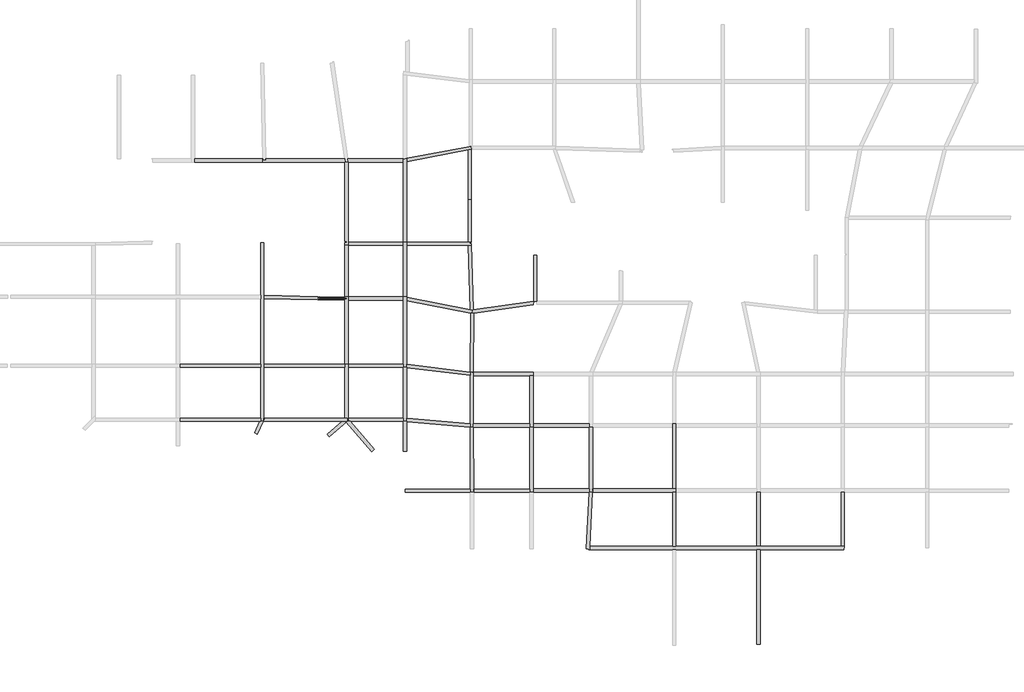
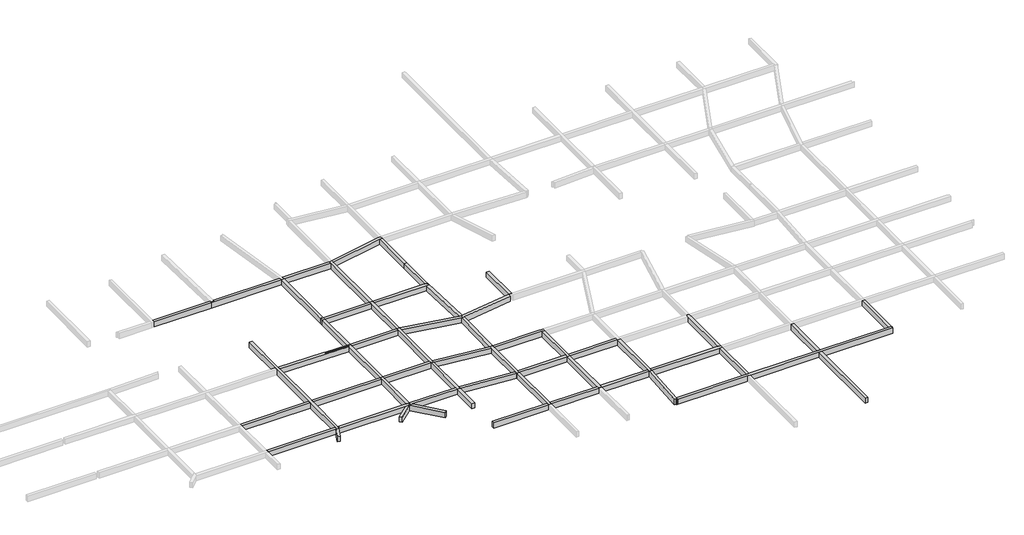
# One storey, part 3 of 15: 55 beams.
"""IFC4 building model written with IfcOpenShell, lengths in millimetres."""

from ifc_helpers import new_model, si_unit, frame, origin, place, context, project, spatial, polyline, outline, extrude, faceted_brep, element, save

model = new_model("IFC4")

# Units and contexts
model_context = context("Model", 3, world=origin())
ifc_project = project(units=[si_unit("LENGTHUNIT", "METRE", prefix="MILLI")], contexts=[model_context])

# Site, building, storey
site = spatial("IfcSite", under=ifc_project)
building = spatial("IfcBuilding", under=site)
storey = spatial("IfcBuildingStorey", under=building, Name="层高", Elevation=3300.0)

# Beams
placement = place(None, origin())
element("IfcBeam", 1, ObjectType="混凝土 - 矩形梁 : KL_beam", at=placement, inside=storey, context=model_context, shape_type="Brep", body=[
    faceted_brep([(134350.2032763, 38806.8951488, 3300.0), (134596.9927787, 38806.8951488, 3300.0), (134650.2032763, 38806.8951488, 3300.0), (134650.2032763, 38924.5535194, 3300.0), (134650.2032763, 39106.8951488, 3300.0), (134650.2032763, 43792.5925365, 3300.0), (134650.2032763, 44092.5925365, 3300.0), (134650.2032763, 50164.3231436, 3300.0), (134650.2032763, 50464.3928831, 3300.0), (134650.2032763, 55332.5925367, 3300.0), (134350.2032763, 55332.5925367, 3300.0), (134350.2032763, 50467.5925366, 3300.0), (134350.2032763, 50167.5925366, 3300.0), (134350.2032763, 44092.5925365, 3300.0), (134350.2032763, 43792.5925365, 3300.0), (134350.2032763, 39106.8951488, 3300.0), (134650.2032763, 38806.8951488, 2700.0), (134650.2032763, 38924.5535194, 2700.0), (134650.2032763, 39106.8951488, 2700.0), (134650.2032763, 43792.5925365, 2700.0), (134650.2032763, 44092.5925365, 2700.0), (134650.2032763, 50164.3231436, 2700.0), (134650.2032763, 50464.3928831, 2700.0), (134650.2032763, 55332.5925367, 2700.0), (134596.9927787, 38806.8951488, 2700.0), (134350.2032763, 38806.8951488, 2700.0), (134350.2032763, 39106.8951488, 2700.0), (134350.2032763, 43792.5925365, 2700.0), (134350.2032763, 44092.5925365, 2700.0), (134350.2032763, 50167.5925366, 2700.0), (134350.2032763, 50467.5925366, 2700.0), (134350.2032763, 55332.5925367, 2700.0)], [[[0, 1, 2, 3, 4, 5, 6, 7, 8, 9, 10, 11, 12, 13, 14, 15]], [[2, 16, 17, 18, 19, 20, 21, 22, 23, 9, 8, 7, 6, 5, 4, 3]], [[16, 24, 25, 26, 27, 28, 29, 30, 31, 23, 22, 21, 20, 19, 18, 17]], [[25, 0, 15, 14, 13, 12, 11, 10, 31, 30, 29, 28, 27, 26]], [[2, 1, 0, 25, 24, 16]], [[10, 9, 23, 31]]]),
])
element("IfcBeam", 2, ObjectType="混凝土 - 矩形梁 : KL_beam", at=placement, inside=storey, context=model_context, shape_type="SweptSolid", body=[
    extrude(outline(polyline([(134350.2032763, 44092.5925365), (134350.2032763, 43792.5925365), (126850.2032763, 43792.5925365), (126850.2032763, 44092.5925365), (134350.2032763, 44092.5925365)])), frame((0.0, 0.0, 2700.0), z_axis=(0.0, 0.0, 1.0), x_axis=(1.0, 0.0, 0.0)), (0.0, 0.0, 1.0), 600.0),
])
element("IfcBeam", 3, ObjectType="混凝土 - 矩形梁 : KL_beam", at=placement, inside=storey, context=model_context, shape_type="Brep", body=[
    faceted_brep([(134350.2032763, 38806.8951488, 3300.0), (134350.2032763, 39106.8951488, 3300.0), (126850.2032763, 39106.8951488, 3300.0), (126850.2032763, 38806.8951488, 3300.0), (134267.7400501, 38806.8951488, 3300.0), (134350.2032763, 38806.8951488, 2700.0), (126850.2032763, 38806.8951488, 2700.0), (134267.7400501, 38806.8951488, 2700.0), (134350.2032763, 39106.8951488, 2700.0), (126850.2032763, 39106.8951488, 2700.0)], [[[0, 1, 2, 3, 4]], [[5, 0, 4, 3, 6, 7]], [[8, 5, 7, 6, 9]], [[1, 8, 9, 2]], [[1, 0, 5, 8]], [[3, 2, 9, 6]]]),
])
element("IfcBeam", 4, ObjectType="混凝土 - 矩形梁 : KL_beam", at=placement, inside=storey, context=model_context, shape_type="Brep", body=[
    faceted_brep([(134060.3828953, 37620.3502485, 3300.0), (133787.0366413, 37743.969929, 3300.0), (133787.0366413, 37743.969929, 2700.0), (134060.3828953, 37620.3502485, 2700.0), (134596.9927787, 38806.8951488, 3300.0), (134350.2032763, 38806.8951488, 3300.0), (134267.7400501, 38806.8951488, 3300.0), (134267.7400501, 38806.8951488, 2700.0), (134350.2032763, 38806.8951488, 2700.0), (134596.9927787, 38806.8951488, 2700.0)], [[[0, 1, 2, 3]], [[1, 0, 4, 5, 6]], [[2, 1, 6, 7]], [[3, 2, 7, 8, 9]], [[0, 3, 9, 4]], [[4, 9, 8, 7, 6, 5]]]),
    faceted_brep([(134650.2032763, 39106.8951488, 2700.0), (134650.2032763, 39106.8951488, 3300.0), (134732.6665025, 39106.8951488, 3300.0), (134732.6665025, 39106.8951488, 2700.0), (134650.2032763, 38924.5535194, 3300.0), (134650.2032763, 38924.5535194, 2700.0)], [[[0, 1, 2, 3]], [[4, 1, 0, 5]], [[4, 2, 1]], [[3, 5, 0]], [[2, 4, 5, 3]]]),
])
element("IfcBeam", 5, ObjectType="混凝土 - 矩形梁 : KL_beam", at=placement, inside=storey, context=model_context, shape_type="Brep", body=[
    faceted_brep([(142355.6857455, 38806.8951488, 3300.0), (142355.6857455, 39106.8951488, 3300.0), (142150.2032763, 39106.8951488, 3300.0), (134732.6665025, 39106.8951488, 3300.0), (134650.2032763, 38924.5535194, 3300.0), (134650.2032763, 38806.8951488, 3300.0), (141894.6697749, 38806.8951488, 3300.0), (142355.6857455, 38806.8951488, 2700.0), (134650.2032763, 38806.8951488, 2700.0), (141894.6697749, 38806.8951488, 2700.0), (142355.6857455, 39106.8951488, 2700.0), (134650.2032763, 38924.5535194, 2700.0), (134732.6665025, 39106.8951488, 2700.0), (142150.2032763, 39106.8951488, 2700.0)], [[[0, 1, 2, 3, 4, 5, 6]], [[7, 0, 6, 5, 8, 9]], [[10, 7, 9, 8, 11, 12, 13]], [[12, 3, 2, 1, 10, 13]], [[3, 12, 11, 4]], [[1, 0, 7, 10]], [[5, 4, 11, 8]]]),
])
element("IfcBeam", 6, ObjectType="混凝土 - 矩形梁 : KL_beam", at=placement, inside=storey, context=model_context, shape_type="SweptSolid", body=[
    extrude(outline(polyline([(140719.4659799, 37404.6255236), (140524.2449773, 37632.4165685), (141894.6697749, 38806.8951488), (142355.6857455, 38806.8951488), (140719.4659799, 37404.6255236)])), frame((0.0, 0.0, 2700.0), z_axis=(0.0, 0.0, 1.0), x_axis=(1.0, 0.0, 0.0)), (0.0, 0.0, 1.0), 600.0),
])
element("IfcBeam", 7, ObjectType="混凝土 - 矩形梁 : KL_beam", at=placement, inside=storey, context=model_context, shape_type="Brep", body=[
    faceted_brep([(142450.2032763, 44092.5925365, 3300.0), (142150.2032763, 44092.5925365, 3300.0), (142150.2032763, 43792.5925365, 3300.0), (142150.2032763, 39106.8951488, 3300.0), (142244.7208071, 39106.8951488, 3300.0), (142355.6857455, 39106.8951488, 3300.0), (142355.6857455, 38806.8951488, 3300.0), (142450.2032763, 38806.8951488, 3300.0), (142450.2032763, 39106.8951488, 3300.0), (142450.2032763, 43792.5925365, 3300.0), (142150.2032763, 39106.8951488, 2700.0), (142150.2032763, 44092.5925365, 2700.0), (142150.2032763, 43792.5925365, 2700.0), (142450.2032763, 44092.5925365, 2700.0), (142450.2032763, 43792.5925365, 2700.0), (142450.2032763, 39106.8951488, 2700.0), (142450.2032763, 38806.8951488, 2700.0), (142355.6857455, 38806.8951488, 2700.0), (142355.6857455, 39106.8951488, 2700.0), (142244.7208071, 39106.8951488, 2700.0)], [[[0, 1, 2, 3, 4, 5, 6, 7, 8, 9]], [[10, 3, 2, 1, 11, 12]], [[11, 13, 14, 15, 16, 17, 18, 19, 10, 12]], [[7, 16, 15, 14, 13, 0, 9, 8]], [[16, 7, 6, 17]], [[3, 10, 19, 18, 5, 4]], [[1, 0, 13, 11]], [[5, 18, 17, 6]]]),
])
element("IfcBeam", 8, ObjectType="混凝土 - 矩形梁 : KL_beam", at=placement, inside=storey, context=model_context, shape_type="SweptSolid", body=[
    extrude(outline(polyline([(142150.2032763, 44092.5925365), (142150.2032763, 43792.5925365), (134650.2032763, 43792.5925365), (134650.2032763, 44092.5925365), (142150.2032763, 44092.5925365)])), frame((0.0, 0.0, 2700.0), z_axis=(0.0, 0.0, 1.0), x_axis=(1.0, 0.0, 0.0)), (0.0, 0.0, 1.0), 600.0),
])
element("IfcBeam", 9, ObjectType="混凝土 - 矩形梁 : KL_beam", at=placement, inside=storey, context=model_context, shape_type="Brep", body=[
    faceted_brep([(142150.2032763, 44092.5925365, 3300.0), (142450.2032763, 44092.5925365, 3300.0), (142450.2032763, 50017.6336553, 3300.0), (142450.2032763, 50317.6336553, 3300.0), (142150.2032763, 50317.6336553, 3300.0), (142150.2032763, 50302.6667178, 3300.0), (142150.2032763, 50227.6336553, 3300.0), (142300.2032763, 50227.6336553, 3300.0), (142300.2032763, 50107.6336553, 3300.0), (142150.2032763, 50107.6336553, 3300.0), (142150.2032763, 50002.5969783, 3300.0), (142450.2032763, 44092.5925365, 2700.0), (142450.2032763, 50017.6336553, 2700.0), (142450.2032763, 50317.6336553, 2700.0), (142150.2032763, 44092.5925365, 2700.0), (142150.2032763, 50002.5969783, 2700.0), (142150.2032763, 50107.6336553, 2700.0), (142300.2032763, 50107.6336553, 2700.0), (142300.2032763, 50227.6336553, 2700.0), (142150.2032763, 50227.6336553, 2700.0), (142150.2032763, 50302.6667178, 2700.0), (142150.2032763, 50317.6336553, 2700.0)], [[[0, 1, 2, 3, 4, 5, 6, 7, 8, 9, 10]], [[1, 11, 12, 13, 3, 2]], [[11, 14, 15, 16, 17, 18, 19, 20, 21, 13, 12]], [[14, 0, 10, 9, 16, 15]], [[1, 0, 14, 11]], [[4, 3, 13, 21]], [[8, 17, 16, 9]], [[18, 7, 6, 19]], [[17, 8, 7, 18]], [[4, 21, 20, 19, 6, 5]]]),
])
element("IfcBeam", 10, ObjectType="混凝土 - 矩形梁 : KL_beam", at=placement, inside=storey, context=model_context, shape_type="SweptSolid", body=[
    extrude(outline(polyline([(139760.2139729, 50227.6336553), (139760.2139729, 50354.2032252), (142150.2032763, 50302.6667178), (142150.2032763, 50227.6336553), (139760.2139729, 50227.6336553)])), frame((0.0, 0.0, 2700.0), z_axis=(0.0, 0.0, 1.0), x_axis=(1.0, 0.0, 0.0)), (0.0, 0.0, 1.0), 600.0),
    extrude(outline(polyline([(134650.2032763, 50164.3231436), (134650.2032763, 50464.3928831), (139640.2139729, 50356.7908438), (139640.2139729, 50107.6336553), (142150.2032763, 50107.6336553), (142150.2032763, 50002.5969783), (134650.2032763, 50164.3231436)])), frame((0.0, 0.0, 2700.0), z_axis=(0.0, 0.0, 1.0), x_axis=(1.0, 0.0, 0.0)), (0.0, 0.0, 1.0), 600.0),
])
element("IfcBeam", 11, ObjectType="混凝土 - 矩形梁 : KL_beam", at=placement, inside=storey, context=model_context, shape_type="Brep", body=[
    faceted_brep([(147550.2032763, 43792.5925365, 3300.0), (147850.2032763, 43792.5925365, 3300.0), (147850.2032763, 44075.472827, 3300.0), (147850.2032763, 49985.080878, 3300.0), (147850.2032763, 50290.8856831, 3300.0), (147850.2032763, 50317.6336548, 3300.0), (147550.2032763, 50317.6336549, 3300.0), (147550.2032763, 50017.6336549, 3300.0), (147550.2032763, 44092.5925365, 3300.0), (147550.2032763, 43792.5925365, 2700.0), (147550.2032763, 50317.6336549, 2700.0), (147550.2032763, 50017.6336549, 2700.0), (147550.2032763, 44092.5925365, 2700.0), (147850.2032763, 43792.5925365, 2700.0), (147850.2032763, 50317.6336548, 2700.0), (147850.2032763, 50290.8856831, 2700.0), (147850.2032763, 49985.080878, 2700.0), (147850.2032763, 44075.472827, 2700.0)], [[[0, 1, 2, 3, 4, 5, 6, 7, 8]], [[9, 0, 8, 7, 6, 10, 11, 12]], [[13, 9, 12, 11, 10, 14, 15, 16, 17]], [[1, 13, 17, 16, 15, 14, 5, 4, 3, 2]], [[1, 0, 9, 13]], [[6, 5, 14, 10]]]),
])
element("IfcBeam", 12, ObjectType="混凝土 - 矩形梁 : KL_beam", at=placement, inside=storey, context=model_context, shape_type="SweptSolid", body=[
    extrude(outline(polyline([(142450.2032763, 43792.5925365), (142450.2032763, 44092.5925365), (147550.2032763, 44092.5925365), (147550.2032763, 43792.5925365), (142450.2032763, 43792.5925365)])), frame((0.0, 0.0, 2700.0), z_axis=(0.0, 0.0, 1.0), x_axis=(1.0, 0.0, 0.0)), (0.0, 0.0, 1.0), 600.0),
])
element("IfcBeam", 13, ObjectType="混凝土 - 矩形梁 : KL_beam", at=placement, inside=storey, context=model_context, shape_type="Brep", body=[
    faceted_brep([(147550.2032763, 38806.8951488, 3300.0), (147850.2032763, 38806.8951488, 3300.0), (147850.2032763, 39094.3896048, 3300.0), (147850.2032763, 43773.2671993, 3300.0), (147850.2032763, 43792.5925365, 3300.0), (147550.2032763, 43792.5925365, 3300.0), (147550.2032763, 39106.8951488, 3300.0), (147550.2032763, 38806.8951488, 2700.0), (147550.2032763, 43792.5925365, 2700.0), (147550.2032763, 39106.8951488, 2700.0), (147850.2032763, 38806.8951488, 2700.0), (147850.2032763, 43792.5925365, 2700.0), (147850.2032763, 43773.2671993, 2700.0), (147850.2032763, 39094.3896048, 2700.0)], [[[0, 1, 2, 3, 4, 5, 6]], [[7, 0, 6, 5, 8, 9]], [[10, 7, 9, 8, 11, 12, 13]], [[1, 10, 13, 12, 11, 4, 3, 2]], [[5, 4, 11, 8]], [[1, 0, 7, 10]]]),
])
element("IfcBeam", 14, ObjectType="混凝土 - 矩形梁 : KL_beam", at=placement, inside=storey, context=model_context, shape_type="Brep", body=[
    faceted_brep([(147550.2032763, 38806.8951488, 3300.0), (147550.2032763, 39106.8951488, 3300.0), (142450.2032763, 39106.8951488, 3300.0), (142450.2032763, 38806.8951488, 3300.0), (142626.6879476, 38806.8951488, 3300.0), (147550.2032763, 38806.8951488, 2700.0), (142450.2032763, 38806.8951488, 2700.0), (142626.6879476, 38806.8951488, 2700.0), (147550.2032763, 39106.8951488, 2700.0), (142450.2032763, 39106.8951488, 2700.0)], [[[0, 1, 2, 3, 4]], [[5, 0, 4, 3, 6, 7]], [[8, 5, 7, 6, 9]], [[1, 8, 9, 2]], [[1, 0, 5, 8]], [[3, 2, 9, 6]]]),
])
element("IfcBeam", 15, ObjectType="混凝土 - 矩形梁 : KL_beam", at=placement, inside=storey, context=model_context, shape_type="Brep", body=[
    faceted_brep([(147850.2032763, 36044.6279155, 3300.0), (147550.2032763, 36044.6279155, 3300.0), (147550.2032763, 36044.6279155, 2700.0), (147850.2032763, 36044.6279155, 2700.0), (147850.2032763, 38793.252187, 3300.0), (147850.2032763, 38806.8951488, 3300.0), (147550.2032763, 38806.8951488, 3300.0), (147550.2032763, 38806.8951488, 2700.0), (147850.2032763, 38806.8951488, 2700.0), (147850.2032763, 38793.252187, 2700.0)], [[[0, 1, 2, 3]], [[1, 0, 4, 5, 6]], [[2, 1, 6, 7]], [[3, 2, 7, 8, 9]], [[0, 3, 9, 8, 5, 4]], [[6, 5, 8, 7]]]),
])
element("IfcBeam", 16, ObjectType="混凝土 - 矩形梁 : KL_beam", at=placement, inside=storey, context=model_context, shape_type="Brep", body=[
    faceted_brep([(144852.3235863, 36214.6134538, 3300.0), (144624.7063393, 36019.1898399, 3300.0), (144624.7063393, 36019.1898399, 2700.0), (144852.3235863, 36214.6134538, 2700.0), (142626.6879476, 38806.8951488, 3300.0), (142450.2032763, 38806.8951488, 3300.0), (142355.6857455, 38806.8951488, 3300.0), (142284.0195543, 38745.4759403, 3300.0), (142284.0195543, 38745.4759403, 2700.0), (142355.6857455, 38806.8951488, 2700.0), (142450.2032763, 38806.8951488, 2700.0), (142626.6879476, 38806.8951488, 2700.0)], [[[0, 1, 2, 3]], [[1, 0, 4, 5, 6, 7]], [[2, 1, 7, 8]], [[3, 2, 8, 9, 10, 11]], [[0, 3, 11, 4]], [[7, 6, 9, 8]], [[4, 11, 10, 9, 6, 5]]]),
])
element("IfcBeam", 17, ObjectType="混凝土 - 矩形梁 : KL_beam", at=placement, inside=storey, context=model_context, shape_type="Brep", body=[
    faceted_brep([(154026.6104044, 43325.1413406, 3300.0), (153885.7263771, 43342.2564237, 3300.0), (153728.3021275, 43361.3808708, 3300.0), (153726.6104044, 43361.5863872, 3300.0), (153726.6104044, 43059.3807595, 3300.0), (153726.6104044, 38582.19205, 3300.0), (153726.6104044, 38281.0546322, 3300.0), (153726.6104044, 38266.5295438, 3300.0), (153727.1862138, 38266.5295438, 3300.0), (154026.6104044, 38266.5295438, 3300.0), (154026.6104044, 38566.5295438, 3300.0), (154026.6104044, 43042.1845858, 3300.0), (154026.6104044, 43325.1413406, 2700.0), (154026.6104044, 38266.5295438, 2700.0), (154026.6104044, 38566.5295438, 2700.0), (154026.6104044, 43042.1845858, 2700.0), (153726.6104044, 43361.5863872, 2700.0), (153728.3021275, 43361.3808708, 2700.0), (153885.7263771, 43342.2564237, 2700.0), (153727.1862138, 38266.5295438, 2700.0), (153726.6104044, 38266.5295438, 2700.0), (153726.6104044, 38281.0546322, 2700.0), (153726.6104044, 38582.19205, 2700.0), (153726.6104044, 43059.3807595, 2700.0)], [[[0, 1, 2, 3, 4, 5, 6, 7, 8, 9, 10, 11]], [[12, 0, 11, 10, 9, 13, 14, 15]], [[16, 17, 18, 12, 15, 14, 13, 19, 20, 21, 22, 23]], [[3, 16, 23, 22, 21, 20, 7, 6, 5, 4]], [[3, 2, 1, 0, 12, 18, 17, 16]], [[9, 8, 7, 20, 19, 13]]]),
])
element("IfcBeam", 18, ObjectType="混凝土 - 矩形梁 : KL_beam", at=placement, inside=storey, context=model_context, shape_type="Brep", body=[
    faceted_brep([(147850.2032763, 44075.472827, 3300.0), (147850.2032763, 43792.5925365, 3300.0), (147850.2032763, 43773.2671993, 3300.0), (153726.6104044, 43059.3807595, 3300.0), (153726.6104044, 43361.5863872, 3300.0), (147850.2032763, 43773.2671993, 2700.0), (153726.6104044, 43059.3807595, 2700.0), (147850.2032763, 43792.5925365, 2700.0), (147850.2032763, 44075.472827, 2700.0), (153726.6104044, 43361.5863872, 2700.0)], [[[0, 1, 2, 3, 4]], [[2, 5, 6, 3]], [[5, 7, 8, 9, 6]], [[8, 0, 4, 9]], [[0, 8, 7, 5, 2, 1]], [[4, 3, 6, 9]]]),
])
element("IfcBeam", 19, ObjectType="混凝土 - 矩形梁 : KL_beam", at=placement, inside=storey, context=model_context, shape_type="Brep", body=[
    faceted_brep([(159549.7804968, 43039.3698021, 3300.0), (159549.7804968, 43042.2492414, 3300.0), (159549.7804968, 43185.5183781, 3300.0), (159549.7804968, 43339.3698411, 3300.0), (159257.4396146, 43339.5188273, 3300.0), (154028.1243818, 43342.1838531, 3300.0), (153885.7263771, 43342.2564237, 3300.0), (154026.6104044, 43325.1413406, 3300.0), (154026.6104044, 43042.1845858, 3300.0), (159248.1480987, 43039.5235236, 3300.0), (159249.7804968, 43039.5226917, 3300.0), (159549.7804968, 43039.3698021, 2700.0), (154026.6104044, 43042.1845858, 2700.0), (159248.1480987, 43039.5235236, 2700.0), (159249.7804968, 43039.5226917, 2700.0), (159549.7804968, 43339.3698411, 2700.0), (159549.7804968, 43185.5183781, 2700.0), (159549.7804968, 43042.2492414, 2700.0), (154026.6104044, 43325.1413406, 2700.0), (153885.7263771, 43342.2564237, 2700.0), (154028.1243818, 43342.1838531, 2700.0), (159257.4396146, 43339.5188273, 2700.0)], [[[0, 1, 2, 3, 4, 5, 6, 7, 8, 9, 10]], [[11, 0, 10, 9, 8, 12, 13, 14]], [[15, 16, 17, 11, 14, 13, 12, 18, 19, 20, 21]], [[3, 15, 21, 20, 19, 6, 5, 4]], [[3, 2, 1, 0, 11, 17, 16, 15]], [[18, 7, 6, 19]], [[7, 18, 12, 8]]]),
])
element("IfcBeam", 20, ObjectType="混凝土 - 矩形梁 : KL_beam", at=placement, inside=storey, context=model_context, shape_type="Brep", body=[
    faceted_brep([(159249.7804968, 38266.5295438, 3300.0), (159549.7804968, 38266.5295438, 3300.0), (159549.7804968, 38566.5295438, 3300.0), (159549.7804968, 43039.3698021, 3300.0), (159249.7804968, 43039.5226917, 3300.0), (159249.7804968, 38566.5295438, 3300.0), (159249.7804968, 38266.5295438, 2700.0), (159249.7804968, 43039.5226917, 2700.0), (159249.7804968, 38566.5295438, 2700.0), (159549.7804968, 38266.5295438, 2700.0), (159549.7804968, 43039.3698021, 2700.0), (159549.7804968, 38566.5295438, 2700.0)], [[[0, 1, 2, 3, 4, 5]], [[6, 0, 5, 4, 7, 8]], [[9, 6, 8, 7, 10, 11]], [[1, 9, 11, 10, 3, 2]], [[4, 3, 10, 7]], [[1, 0, 6, 9]]]),
])
element("IfcBeam", 21, ObjectType="混凝土 - 矩形梁 : KL_beam", at=placement, inside=storey, context=model_context, shape_type="Brep", body=[
    faceted_brep([(159249.7804968, 38266.5295438, 3300.0), (159249.7804968, 38566.5295438, 3300.0), (154026.6104044, 38566.5295438, 3300.0), (154026.6104044, 38266.5295438, 3300.0), (154027.1884327, 38266.5295438, 3300.0), (159249.7804968, 38266.5295438, 2700.0), (154026.6104044, 38266.5295438, 2700.0), (154027.1884327, 38266.5295438, 2700.0), (159249.7804968, 38566.5295438, 2700.0), (154026.6104044, 38566.5295438, 2700.0)], [[[0, 1, 2, 3, 4]], [[5, 0, 4, 3, 6, 7]], [[8, 5, 7, 6, 9]], [[1, 8, 9, 2]], [[1, 0, 5, 8]], [[3, 2, 9, 6]]]),
])
element("IfcBeam", 22, ObjectType="混凝土 - 矩形梁 : KL_beam", at=placement, inside=storey, context=model_context, shape_type="Brep", body=[
    faceted_brep([(153750.3563062, 32242.26105, 3300.0), (154050.3540873, 32243.4148791, 3300.0), (154049.7804968, 32392.5495084, 3300.0), (154049.2046874, 32542.26105, 3300.0), (154027.1884327, 38266.5295438, 3300.0), (154026.6104044, 38266.5295438, 3300.0), (153727.1862138, 38266.5295438, 3300.0), (153749.2024685, 32542.26105, 3300.0), (154050.3540873, 32243.4148791, 2700.0), (154049.7804968, 32392.5495084, 2700.0), (154049.2046874, 32542.26105, 2700.0), (154027.1884327, 38266.5295438, 2700.0), (153750.3563062, 32242.26105, 2700.0), (153749.2024685, 32542.26105, 2700.0), (153727.1862138, 38266.5295438, 2700.0), (154026.6104044, 38266.5295438, 2700.0)], [[[0, 1, 2, 3, 4, 5, 6, 7]], [[1, 8, 9, 10, 11, 4, 3, 2]], [[8, 12, 13, 14, 15, 11, 10, 9]], [[12, 0, 7, 6, 14, 13]], [[6, 5, 4, 11, 15, 14]], [[0, 12, 8, 1]]]),
])
element("IfcBeam", 23, ObjectType="混凝土 - 矩形梁 : KL_beam", at=placement, inside=storey, context=model_context, shape_type="Brep", body=[
    faceted_brep([(147748.4611459, 32242.26105, 3300.0), (147748.4611459, 32542.26105, 3300.0), (147748.4611459, 32542.26105, 2700.0), (147748.4611459, 32242.26105, 2700.0), (153749.7804968, 32242.26105, 3300.0), (153750.3563062, 32242.26105, 3300.0), (153749.2024685, 32542.26105, 3300.0), (153749.2024685, 32542.26105, 2700.0), (153750.3563062, 32242.26105, 2700.0), (153749.7804968, 32242.26105, 2700.0), (154049.7804968, 32242.26105, 2700.0), (154050.3585251, 32242.26105, 2700.0), (154050.3585251, 32242.26105, 3300.0), (154049.7804968, 32242.26105, 3300.0), (154050.3540873, 32243.4148791, 2700.0), (154050.3540873, 32243.4148791, 3300.0)], [[[0, 1, 2, 3]], [[1, 0, 4, 5, 6]], [[2, 1, 6, 7]], [[3, 2, 7, 8, 9]], [[0, 3, 9, 8, 10, 11, 12, 13, 5, 4]], [[5, 8, 7, 6]], [[12, 11, 14, 15]], [[8, 5, 15, 14]], [[5, 13, 12, 15]], [[14, 11, 10, 8]]]),
])
element("IfcBeam", 24, ObjectType="混凝土 - 矩形梁 : KL_beam", at=placement, inside=storey, context=model_context, shape_type="SweptSolid", body=[
    extrude(outline(polyline([(142450.2032763, 50017.6336553), (142450.2032763, 50317.6336553), (147550.2032763, 50317.6336549), (147550.2032763, 50017.6336549), (142450.2032763, 50017.6336553)])), frame((0.0, 0.0, 2700.0), z_axis=(0.0, 0.0, 1.0), x_axis=(1.0, 0.0, 0.0)), (0.0, 0.0, 1.0), 600.0),
])
element("IfcBeam", 25, ObjectType="混凝土 - 矩形梁 : KL_beam", at=placement, inside=storey, context=model_context, shape_type="Brep", body=[
    faceted_brep([(147850.2032738, 55392.5925366, 3300.0), (147550.2032738, 55392.5925366, 3300.0), (147550.2032738, 55382.5925365, 3300.0), (147550.203274, 55082.5925365, 3300.0), (147550.2032762, 50317.6336549, 3300.0), (147850.2032762, 50317.6336548, 3300.0), (147850.203274, 55092.5925366, 3300.0), (147550.2032738, 55392.5925366, 2700.0), (147550.2032738, 55382.5925365, 2700.0), (147550.203274, 55082.5925365, 2700.0), (147550.2032762, 50317.6336549, 2700.0), (147850.2032738, 55392.5925366, 2700.0), (147850.203274, 55092.5925366, 2700.0), (147850.2032762, 50317.6336548, 2700.0)], [[[0, 1, 2, 3, 4, 5, 6]], [[1, 7, 8, 9, 10, 4, 3, 2]], [[7, 11, 12, 13, 10, 9, 8]], [[11, 0, 6, 5, 13, 12]], [[1, 0, 11, 7]], [[5, 4, 10, 13]]]),
])
element("IfcBeam", 26, ObjectType="混凝土 - 矩形梁 : KL_beam", at=placement, inside=storey, context=model_context, shape_type="Brep", body=[
    faceted_brep([(153895.7696272, 48790.0588433, 3300.0), (153903.7913665, 49094.2779979, 3300.0), (153721.7041547, 49130.2710244, 3300.0), (147850.2032762, 50290.8856831, 3300.0), (147850.2032762, 50017.6336548, 3300.0), (147850.2032763, 49985.080878, 3300.0), (153783.0726395, 48812.3355624, 3300.0), (147850.2032763, 49985.080878, 2700.0), (153783.0726395, 48812.3355624, 2700.0), (153895.7696272, 48790.0588433, 2700.0), (153903.7913665, 49094.2779979, 2700.0), (147850.2032762, 50017.6336548, 2700.0), (147850.2032762, 50290.8856831, 2700.0), (153721.7041547, 49130.2710244, 2700.0)], [[[0, 1, 2, 3, 4, 5, 6]], [[5, 7, 8, 9, 0, 6]], [[10, 9, 8, 7, 11, 12, 13]], [[12, 3, 2, 1, 10, 13]], [[3, 12, 11, 7, 5, 4]], [[1, 0, 9, 10]]]),
])
element("IfcBeam", 27, ObjectType="混凝土 - 矩形梁 : KL_beam", at=placement, inside=storey, context=model_context, shape_type="Brep", body=[
    faceted_brep([(147850.2032738, 55392.5925366, 3300.0), (147850.203274, 55092.5925366, 3300.0), (153554.4497163, 55092.5925366, 3300.0), (153850.3009381, 55092.5925366, 3300.0), (153850.3009381, 55244.6960153, 3300.0), (153850.3009381, 55257.9423641, 3300.0), (153700.298991, 55257.9423641, 3300.0), (153700.298991, 55377.9423641, 3300.0), (153850.3009381, 55377.9423641, 3300.0), (153850.3009381, 55392.5925366, 3300.0), (153550.3009381, 55392.5925366, 3300.0), (153850.3009381, 55092.5925366, 2700.0), (147850.203274, 55092.5925366, 2700.0), (153554.4497163, 55092.5925366, 2700.0), (147850.2032738, 55392.5925366, 2700.0), (153550.3009381, 55392.5925366, 2700.0), (153850.3009381, 55392.5925366, 2700.0), (153850.3009381, 55377.9423641, 2700.0), (153700.298991, 55377.9423641, 2700.0), (153700.298991, 55257.9423641, 2700.0), (153850.3009381, 55257.9423641, 2700.0), (153850.3009381, 55244.6960153, 2700.0)], [[[0, 1, 2, 3, 4, 5, 6, 7, 8, 9, 10]], [[11, 3, 2, 1, 12, 13]], [[12, 14, 15, 16, 17, 18, 19, 20, 21, 11, 13]], [[9, 16, 15, 14, 0, 10]], [[16, 9, 8, 17]], [[1, 0, 14, 12]], [[7, 18, 17, 8]], [[19, 6, 5, 20]], [[18, 7, 6, 19]], [[3, 11, 21, 20, 5, 4]]]),
])
element("IfcBeam", 28, ObjectType="混凝土 - 矩形梁 : KL_beam", at=placement, inside=storey, context=model_context, shape_type="SweptSolid", body=[
    extrude(outline(polyline([(153550.3009381, 59292.1684205), (153850.3009381, 59292.1684205), (153850.3009381, 55392.5925366), (153550.3009381, 55392.5925366), (153550.3009381, 59292.1684205)])), frame((0.0, 0.0, 2700.0), z_axis=(0.0, 0.0, 1.0), x_axis=(1.0, 0.0, 0.0)), (0.0, 0.0, 1.0), 600.0),
])
element("IfcBeam", 29, ObjectType="混凝土 - 矩形梁 : KL_beam", at=placement, inside=storey, context=model_context, shape_type="Brep", body=[
    faceted_brep([(147850.2032739, 63124.0584778, 3300.0), (147550.2032739, 63066.5805581, 3300.0), (147550.2032739, 62792.591237, 3300.0), (147550.2032739, 55392.5925366, 3300.0), (147850.2032739, 55392.5925366, 3300.0), (147850.2032739, 62818.6019158, 3300.0), (147850.2032739, 63124.0584778, 2700.0), (147850.2032739, 55392.5925366, 2700.0), (147850.2032739, 62818.6019158, 2700.0), (147550.2032739, 63066.5805581, 2700.0), (147550.2032739, 55392.5925366, 2700.0), (147550.2032739, 62792.591237, 2700.0)], [[[0, 1, 2, 3, 4, 5]], [[6, 0, 5, 4, 7, 8]], [[9, 6, 8, 7, 10, 11]], [[1, 9, 11, 10, 3, 2]], [[4, 3, 10, 7]], [[1, 0, 6, 9]]]),
])
element("IfcBeam", 30, ObjectType="混凝土 - 矩形梁 : KL_beam", at=placement, inside=storey, context=model_context, shape_type="Brep", body=[
    faceted_brep([(153850.3013477, 63968.1790994, 3300.0), (153793.8501921, 64262.8200114, 3300.0), (153625.2394262, 64230.5153579, 3300.0), (147850.2032739, 63124.0584778, 3300.0), (147850.2032739, 62818.6019158, 3300.0), (153550.3013477, 63910.7011797, 3300.0), (153793.8501921, 64262.8200114, 2700.0), (153625.2394262, 64230.5153579, 2700.0), (147850.2032739, 63124.0584778, 2700.0), (153850.3013477, 63968.1790994, 2700.0), (153550.3013477, 63910.7011797, 2700.0), (147850.2032739, 62818.6019158, 2700.0)], [[[0, 1, 2, 3, 4, 5]], [[1, 6, 7, 8, 3, 2]], [[6, 9, 10, 11, 8, 7]], [[9, 0, 5, 4, 11, 10]], [[4, 3, 8, 11]], [[0, 9, 6, 1]]]),
])
element("IfcBeam", 31, ObjectType="混凝土 - 矩形梁 : KL_beam", at=placement, inside=storey, context=model_context, shape_type="Brep", body=[
    faceted_brep([(153850.3013477, 59292.1684205, 3300.0), (153850.3013477, 63956.5260367, 3300.0), (153850.3013477, 63968.1790994, 3300.0), (153550.3013477, 63910.7011797, 3300.0), (153550.3013477, 59292.1684205, 3300.0), (153550.3013477, 59292.1684205, 2700.0), (153550.3013477, 63910.7011797, 2700.0), (153850.3013477, 63968.1790994, 2700.0), (153850.3013477, 63956.5260367, 2700.0), (153850.3013477, 59292.1684205, 2700.0)], [[[0, 1, 2, 3, 4]], [[5, 4, 3, 6]], [[7, 8, 9, 5, 6]], [[2, 1, 0, 9, 8, 7]], [[0, 4, 5, 9]], [[3, 2, 7, 6]]]),
])
element("IfcBeam", 32, ObjectType="混凝土 - 矩形梁 : KL_beam", at=placement, inside=storey, context=model_context, shape_type="SweptSolid", body=[
    extrude(outline(polyline([(159549.7804968, 38266.5295438), (159549.7804968, 38566.5295438), (164749.7804968, 38566.5295438), (164749.7804968, 38266.5295438), (159549.7804968, 38266.5295438)])), frame((0.0, 0.0, 2700.0), z_axis=(0.0, 0.0, 1.0), x_axis=(1.0, 0.0, 0.0)), (0.0, 0.0, 1.0), 600.0),
])
element("IfcBeam", 33, ObjectType="混凝土 - 矩形梁 : KL_beam", at=placement, inside=storey, context=model_context, shape_type="Brep", body=[
    faceted_brep([(164749.7804968, 32266.5295438, 3300.0), (165042.5880282, 32266.5295438, 3300.0), (165049.7804968, 32266.5295438, 3300.0), (165049.7804968, 32412.8449723, 3300.0), (165049.7804968, 32566.5295438, 3300.0), (165049.7804968, 38266.5295438, 3300.0), (164749.7804968, 38266.5295438, 3300.0), (164749.7804968, 32566.5295438, 3300.0), (164749.7804968, 32266.5295438, 2700.0), (164749.7804968, 38266.5295438, 2700.0), (164749.7804968, 32566.5295438, 2700.0), (165049.7804968, 32266.5295438, 2700.0), (165042.5880282, 32266.5295438, 2700.0), (165049.7804968, 38266.5295438, 2700.0), (165049.7804968, 32566.5295438, 2700.0), (165049.7804968, 32412.8449723, 2700.0)], [[[0, 1, 2, 3, 4, 5, 6, 7]], [[8, 0, 7, 6, 9, 10]], [[11, 12, 8, 10, 9, 13, 14, 15]], [[2, 11, 15, 14, 13, 5, 4, 3]], [[6, 5, 13, 9]], [[2, 1, 0, 8, 12, 11]]]),
])
element("IfcBeam", 34, ObjectType="混凝土 - 矩形梁 : KL_beam", at=placement, inside=storey, context=model_context, shape_type="Brep", body=[
    faceted_brep([(159249.7804968, 32266.5295438, 3300.0), (159549.7804968, 32266.5295438, 3300.0), (159549.7804968, 32566.5295438, 3300.0), (159549.7804968, 38266.5295438, 3300.0), (159249.7804968, 38266.5295438, 3300.0), (159249.7804968, 32542.26105, 3300.0), (159249.7804968, 32266.5295438, 2700.0), (159249.7804968, 38266.5295438, 2700.0), (159249.7804968, 32542.26105, 2700.0), (159549.7804968, 32266.5295438, 2700.0), (159549.7804968, 38266.5295438, 2700.0), (159549.7804968, 32566.5295438, 2700.0)], [[[0, 1, 2, 3, 4, 5]], [[6, 0, 5, 4, 7, 8]], [[9, 6, 8, 7, 10, 11]], [[1, 9, 11, 10, 3, 2]], [[4, 3, 10, 7]], [[1, 0, 6, 9]]]),
])
element("IfcBeam", 35, ObjectType="混凝土 - 矩形梁 : KL_beam", at=placement, inside=storey, context=model_context, shape_type="Brep", body=[
    faceted_brep([(164749.7804968, 32266.5295438, 3300.0), (164749.7804968, 32566.5295438, 3300.0), (159549.7804968, 32566.5295438, 3300.0), (159549.7804968, 32266.5295438, 3300.0), (164742.2257811, 32266.5295438, 3300.0), (164749.7804968, 32266.5295438, 2700.0), (159549.7804968, 32266.5295438, 2700.0), (164742.2257811, 32266.5295438, 2700.0), (164749.7804968, 32566.5295438, 2700.0), (159549.7804968, 32566.5295438, 2700.0)], [[[0, 1, 2, 3, 4]], [[5, 0, 4, 3, 6, 7]], [[8, 5, 7, 6, 9]], [[1, 8, 9, 2]], [[1, 0, 5, 8]], [[3, 2, 9, 6]]]),
])
element("IfcBeam", 36, ObjectType="混凝土 - 矩形梁 : KL_beam", at=placement, inside=storey, context=model_context, shape_type="Brep", body=[
    faceted_brep([(159549.7804968, 32242.26105, 2700.0), (159549.7804968, 32242.26105, 3300.0), (159249.7804968, 32242.26105, 3300.0), (154050.3585251, 32242.26105, 3300.0), (154050.3585251, 32242.26105, 2700.0), (159249.7804968, 32242.26105, 2700.0), (159249.7804968, 32542.26105, 3300.0), (159249.7804968, 32542.26105, 2700.0), (154049.7804968, 32542.26105, 2700.0), (154049.7804968, 32542.26105, 3300.0), (159549.7804968, 32266.5295438, 2700.0), (159549.7804968, 32266.5295438, 3300.0), (154049.7804968, 32392.5495084, 3300.0), (154049.7804968, 32392.5495084, 2700.0), (154050.3540873, 32243.4148791, 2700.0), (154050.3540873, 32243.4148791, 3300.0), (159249.7804968, 32266.5295438, 3300.0), (159249.7804968, 32266.5295438, 2700.0)], [[[0, 1, 2, 3, 4, 5]], [[6, 7, 8, 9]], [[1, 0, 10, 11]], [[12, 13, 14, 4, 3, 15]], [[13, 12, 9, 8]], [[16, 17, 7, 6]], [[17, 16, 11, 10]], [[1, 11, 16, 6, 9, 12, 15, 3, 2]], [[10, 0, 5, 4, 14, 13, 8, 7, 17]]]),
])
element("IfcBeam", 37, ObjectType="混凝土 - 矩形梁 : KL_beam", at=placement, inside=storey, context=model_context, shape_type="Brep", body=[
    faceted_brep([(165042.5880282, 32266.5295438, 3300.0), (164749.7804968, 32266.5295438, 3300.0), (164742.2257811, 32266.5295438, 3300.0), (164485.5488101, 27044.9842098, 3300.0), (164692.7804968, 27044.9842098, 3300.0), (164692.7804968, 26924.9842098, 3300.0), (164780.0121835, 26924.9842098, 3300.0), (164780.861466, 26942.26105, 3300.0), (164795.6086502, 27242.26105, 3300.0), (164742.2257811, 32266.5295438, 2700.0), (164485.5488101, 27044.9842098, 2700.0), (164749.7804968, 32266.5295438, 2700.0), (165042.5880282, 32266.5295438, 2700.0), (164795.6086502, 27242.26105, 2700.0), (164780.861466, 26942.26105, 2700.0), (164780.0121835, 26924.9842098, 2700.0), (164692.7804968, 26924.9842098, 2700.0), (164692.7804968, 27044.9842098, 2700.0)], [[[0, 1, 2, 3, 4, 5, 6, 7, 8]], [[2, 9, 10, 3]], [[9, 11, 12, 13, 14, 15, 16, 17, 10]], [[12, 0, 8, 7, 6, 15, 14, 13]], [[0, 12, 11, 9, 2, 1]], [[15, 6, 5, 16]], [[17, 4, 3, 10]], [[4, 17, 16, 5]]]),
    faceted_brep([(165049.7804968, 32566.5295438, 2700.0), (165049.7804968, 32566.5295438, 3300.0), (165057.3352125, 32566.5295438, 3300.0), (165057.3352125, 32566.5295438, 2700.0), (165049.7804968, 32412.8449723, 3300.0), (165049.7804968, 32412.8449723, 2700.0)], [[[0, 1, 2, 3]], [[4, 1, 0, 5]], [[1, 4, 2]], [[5, 0, 3]], [[4, 5, 3, 2]]]),
])
element("IfcBeam", 38, ObjectType="混凝土 - 矩形梁 : KL_beam", at=placement, inside=storey, context=model_context, shape_type="Brep", body=[
    faceted_brep([(172749.7804968, 32566.5295438, 3300.0), (172749.7804968, 32566.5295438, 2700.0), (172449.7804968, 32566.5295438, 2700.0), (165057.3352125, 32566.5295438, 2700.0), (165057.3352125, 32566.5295438, 3300.0), (172449.7804968, 32566.5295438, 3300.0), (165049.7804968, 32266.5295438, 2700.0), (165049.7804968, 32266.5295438, 3300.0), (165049.7804968, 32412.8449723, 3300.0), (165049.7804968, 32412.8449723, 2700.0), (172749.7804968, 32266.5295438, 3300.0), (172449.7804968, 32266.5295438, 3300.0), (172449.7804968, 32266.5295438, 2700.0), (172749.7804968, 32266.5295438, 2700.0)], [[[0, 1, 2, 3, 4, 5]], [[6, 7, 8, 9]], [[10, 0, 5, 4, 8, 7, 11]], [[7, 6, 12, 13, 10, 11]], [[1, 13, 12, 6, 9, 3, 2]], [[4, 3, 9, 8]], [[0, 10, 13, 1]]]),
])
element("IfcBeam", 39, ObjectType="混凝土 - 矩形梁 : KL_beam", at=placement, inside=storey, context=model_context, shape_type="Brep", body=[
    faceted_brep([(172749.7804968, 38566.5295438, 3300.0), (172449.7804968, 38566.5295438, 3300.0), (172449.7804968, 38266.5295438, 3300.0), (172449.7804968, 32566.5295438, 3300.0), (172749.7804968, 32566.5295438, 3300.0), (172749.7804968, 38266.5295438, 3300.0), (172749.7804968, 38566.5295438, 2700.0), (172749.7804968, 32566.5295438, 2700.0), (172749.7804968, 38266.5295438, 2700.0), (172449.7804968, 38566.5295438, 2700.0), (172449.7804968, 32566.5295438, 2700.0), (172449.7804968, 38266.5295438, 2700.0)], [[[0, 1, 2, 3, 4, 5]], [[6, 0, 5, 4, 7, 8]], [[9, 6, 8, 7, 10, 11]], [[1, 9, 11, 10, 3, 2]], [[4, 3, 10, 7]], [[1, 0, 6, 9]]]),
])
element("IfcBeam", 40, ObjectType="混凝土 - 矩形梁 : KL_beam", at=placement, inside=storey, context=model_context, shape_type="SweptSolid", body=[
    extrude(outline(polyline([(172449.7804968, 32266.5295438), (172749.7804968, 32266.5295438), (172749.7804968, 27242.26105), (172449.7804968, 27242.26105), (172449.7804968, 32266.5295438)])), frame((0.0, 0.0, 2700.0), z_axis=(0.0, 0.0, 1.0), x_axis=(1.0, 0.0, 0.0)), (0.0, 0.0, 1.0), 600.0),
])
element("IfcBeam", 41, ObjectType="混凝土 - 矩形梁 : KL_beam", at=placement, inside=storey, context=model_context, shape_type="SweptSolid", body=[
    extrude(outline(polyline([(180249.7804968, 32266.5295438), (180549.7804968, 32266.5295438), (180549.7804968, 27242.26105), (180249.7804968, 27242.26105), (180249.7804968, 32266.5295438)])), frame((0.0, 0.0, 2700.0), z_axis=(0.0, 0.0, 1.0), x_axis=(1.0, 0.0, 0.0)), (0.0, 0.0, 1.0), 600.0),
])
element("IfcBeam", 42, ObjectType="混凝土 - 矩形梁 : KL_beam", at=placement, inside=storey, context=model_context, shape_type="Brep", body=[
    faceted_brep([(159601.8562875, 49911.380442, 3300.0), (159595.197808, 49910.4256161, 3300.0), (154022.3549019, 49111.2800075, 3300.0), (153903.7913665, 49094.2779979, 3300.0), (153895.7696272, 48790.0588433, 3300.0), (154083.1339161, 48816.9268802, 3300.0), (159585.8528526, 49606.0167123, 3300.0), (159601.8562875, 49911.380442, 2700.0), (159595.197808, 49910.4256161, 2700.0), (154022.3549019, 49111.2800075, 2700.0), (153903.7913665, 49094.2779979, 2700.0), (159585.8528526, 49606.0167123, 2700.0), (154083.1339161, 48816.9268802, 2700.0), (153895.7696272, 48790.0588433, 2700.0)], [[[0, 1, 2, 3, 4, 5, 6]], [[3, 2, 1, 0, 7, 8, 9, 10]], [[10, 9, 8, 7, 11, 12, 13]], [[11, 6, 5, 4, 13, 12]], [[0, 6, 11, 7]], [[4, 3, 10, 13]]]),
])
element("IfcBeam", 43, ObjectType="混凝土 - 矩形梁 : KL_beam", at=placement, inside=storey, context=model_context, shape_type="SweptSolid", body=[
    extrude(outline(polyline([(159601.8562875, 49911.380442), (159595.197808, 49910.4256161), (159595.197808, 54181.7848082), (159895.197808, 54181.7848082), (159895.197808, 49930.4011957), (159602.853123, 49930.4011957), (159601.8562875, 49911.380442)])), frame((0.0, 0.0, 2700.0), z_axis=(0.0, 0.0, 1.0), x_axis=(1.0, 0.0, 0.0)), (0.0, 0.0, 1.0), 600.0),
])
element("IfcBeam", 44, ObjectType="混凝土 - 矩形梁 : KL_beam", at=placement, inside=storey, context=model_context, shape_type="Brep", body=[
    faceted_brep([(147850.2032763, 38793.252187, 3300.0), (147850.2032763, 38793.252187, 2700.0), (153726.6104044, 38281.0546322, 2700.0), (153726.6104044, 38281.0546322, 3300.0), (147850.2032763, 39094.3896048, 3300.0), (147850.2032763, 39094.3896048, 2700.0), (147850.2032763, 38806.8951488, 2700.0), (147850.2032763, 38806.8951488, 3300.0), (153726.6104044, 38582.19205, 2700.0), (153726.6104044, 38582.19205, 3300.0)], [[[0, 1, 2, 3]], [[4, 5, 6, 1, 0, 7]], [[3, 2, 8, 9]], [[4, 7, 0, 3, 9]], [[1, 6, 5, 8, 2]], [[5, 4, 9, 8]]]),
])
element("IfcBeam", 45, ObjectType="混凝土 - 矩形梁 : KL_beam", at=placement, inside=storey, context=model_context, shape_type="SweptSolid", body=[
    extrude(outline(polyline([(180549.7804968, 18192.1825093), (180249.7804968, 18192.1825093), (180249.7804968, 26942.26105), (180549.7804968, 26942.26105), (180549.7804968, 18192.1825093)])), frame((0.0, 0.0, 2700.0), z_axis=(0.0, 0.0, 1.0), x_axis=(1.0, 0.0, 0.0)), (0.0, 0.0, 1.0), 600.0),
])
element("IfcBeam", 46, ObjectType="混凝土 - 矩形梁 : KL_beam", at=placement, inside=storey, context=model_context, shape_type="Brep", body=[
    faceted_brep([(164795.6086502, 27242.26105, 3300.0), (164780.861466, 26942.26105, 3300.0), (172449.7804968, 26942.26105, 3300.0), (172749.7804968, 26942.26105, 3300.0), (180249.7804968, 26942.26105, 3300.0), (180549.7804968, 26942.26105, 3300.0), (188304.7804971, 26942.26105, 3300.0), (188304.7804971, 27102.1039685, 3300.0), (188349.7804968, 27102.1039685, 3300.0), (188349.7804968, 27242.26105, 3300.0), (188049.7804968, 27242.26105, 3300.0), (180549.7804968, 27242.26105, 3300.0), (180249.7804968, 27242.26105, 3300.0), (172749.7804968, 27242.26105, 3300.0), (172449.7804968, 27242.26105, 3300.0), (164780.861466, 26942.26105, 2700.0), (172449.7804968, 26942.26105, 2700.0), (172749.7804968, 26942.26105, 2700.0), (180249.7804968, 26942.26105, 2700.0), (180549.7804968, 26942.26105, 2700.0), (188304.7804971, 26942.26105, 2700.0), (164795.6086502, 27242.26105, 2700.0), (172449.7804968, 27242.26105, 2700.0), (172749.7804968, 27242.26105, 2700.0), (180249.7804968, 27242.26105, 2700.0), (180549.7804968, 27242.26105, 2700.0), (188049.7804968, 27242.26105, 2700.0), (188349.7804968, 27242.26105, 2700.0), (188349.7804968, 27102.1039685, 2700.0), (188304.7804971, 27102.1039685, 2700.0)], [[[0, 1, 2, 3, 4, 5, 6, 7, 8, 9, 10, 11, 12, 13, 14]], [[1, 15, 16, 17, 18, 19, 20, 6, 5, 4, 3, 2]], [[15, 21, 22, 23, 24, 25, 26, 27, 28, 29, 20, 19, 18, 17, 16]], [[21, 0, 14, 13, 12, 11, 10, 9, 27, 26, 25, 24, 23, 22]], [[1, 0, 21, 15]], [[27, 9, 8, 28]], [[29, 7, 6, 20]], [[7, 29, 28, 8]]]),
])
element("IfcBeam", 47, ObjectType="混凝土 - 矩形梁 : KL_beam", at=placement, inside=storey, context=model_context, shape_type="SweptSolid", body=[
    extrude(outline(polyline([(188049.7804968, 32266.5295438), (188349.7804968, 32266.5295438), (188349.7804968, 27242.26105), (188049.7804968, 27242.26105), (188049.7804968, 32266.5295438)])), frame((0.0, 0.0, 2700.0), z_axis=(0.0, 0.0, 1.0), x_axis=(1.0, 0.0, 0.0)), (0.0, 0.0, 1.0), 600.0),
])
element("IfcBeam", 48, ObjectType="混凝土 - 矩形梁 : KL_beam", at=placement, inside=storey, context=model_context, shape_type="Brep", body=[
    faceted_brep([(142429.4864877, 63092.591237, 3300.0), (142474.2397946, 62792.591237, 3300.0), (147550.2032739, 62792.591237, 3300.0), (147550.203276, 63066.5805581, 3300.0), (147550.2032763, 63092.591237, 3300.0), (142474.2397946, 62792.591237, 2700.0), (147550.2032739, 62792.591237, 2700.0), (142429.4864877, 63092.591237, 2700.0), (147550.2032763, 63092.591237, 2700.0), (147550.203276, 63066.5805581, 2700.0)], [[[0, 1, 2, 3, 4]], [[1, 5, 6, 2]], [[5, 7, 8, 9, 6]], [[7, 0, 4, 8]], [[1, 0, 7, 5]], [[2, 6, 9, 8, 4, 3]]]),
])
element("IfcBeam", 49, ObjectType="混凝土 - 矩形梁 : KL_beam", at=placement, inside=storey, context=model_context, shape_type="SweptSolid", body=[
    extrude(outline(polyline([(134500.2032763, 63092.591237), (134500.2032763, 62792.591237), (128250.8470615, 62792.591237), (128250.8470615, 63092.591237), (134500.2032763, 63092.591237)])), frame((0.0, 0.0, 2700.0), z_axis=(0.0, 0.0, 1.0), x_axis=(1.0, 0.0, 0.0)), (0.0, 0.0, 1.0), 600.0),
])
element("IfcBeam", 50, ObjectType="混凝土 - 矩形梁 : KL_beam", at=placement, inside=storey, context=model_context, shape_type="Brep", body=[
    faceted_brep([(134500.2032763, 63092.591237, 3300.0), (134500.2032763, 62792.591237, 3300.0), (142150.2032763, 62792.591237, 3300.0), (142170.9200648, 62792.591237, 3300.0), (142126.1667579, 63092.591237, 3300.0), (134846.9249344, 63092.591237, 3300.0), (134850.1658492, 62945.9420507, 3300.0), (134550.2390825, 62939.313735, 3300.0), (134546.8516833, 63092.591237, 3300.0), (134500.2032763, 62792.591237, 2700.0), (142150.2032763, 62792.591237, 2700.0), (142170.9200648, 62792.591237, 2700.0), (134500.2032763, 63092.591237, 2700.0), (134546.8516833, 63092.591237, 2700.0), (134550.2390825, 62939.313735, 2700.0), (134850.1658492, 62945.9420507, 2700.0), (134846.9249344, 63092.591237, 2700.0), (142126.1667579, 63092.591237, 2700.0)], [[[0, 1, 2, 3, 4, 5, 6, 7, 8]], [[1, 9, 10, 11, 3, 2]], [[9, 12, 13, 14, 15, 16, 17, 11, 10]], [[4, 17, 16, 5]], [[0, 12, 9, 1]], [[4, 3, 11, 17]], [[14, 7, 6, 15]], [[15, 6, 5, 16]], [[7, 14, 13, 8]], [[12, 0, 8, 13]]]),
])
element("IfcBeam", 51, ObjectType="混凝土 - 矩形梁 : KL_beam", at=placement, inside=storey, context=model_context, shape_type="SweptSolid", body=[
    extrude(outline(polyline([(153554.4497163, 55092.5925366), (153850.3009381, 55092.5925366), (153850.3009381, 55244.6960153), (154022.3549019, 49111.2800075), (153903.7913665, 49094.2779979), (153721.7041547, 49130.2710244), (153554.4497163, 55092.5925366)])), frame((0.0, 0.0, 2700.0), z_axis=(0.0, 0.0, 1.0), x_axis=(1.0, 0.0, 0.0)), (0.0, 0.0, 1.0), 600.0),
])
element("IfcBeam", 52, ObjectType="混凝土 - 矩形梁 : KL_beam", at=placement, inside=storey, context=model_context, shape_type="Brep", body=[
    faceted_brep([(153728.3021275, 43361.3808708, 3300.0), (153885.7263771, 43342.2564237, 3300.0), (154028.1243818, 43342.1838531, 3300.0), (154083.1339161, 48816.9268802, 3300.0), (154030.8224961, 48809.4254232, 3300.0), (153895.7696272, 48790.0588433, 3300.0), (153783.0726395, 48812.3355624, 3300.0), (154028.1243818, 43342.1838531, 2700.0), (154083.1339161, 48816.9268802, 2700.0), (153885.7263771, 43342.2564237, 2700.0), (153728.3021275, 43361.3808708, 2700.0), (153783.0726395, 48812.3355624, 2700.0), (153895.7696272, 48790.0588433, 2700.0), (154030.8224961, 48809.4254232, 2700.0)], [[[0, 1, 2, 3, 4, 5, 6]], [[2, 7, 8, 3]], [[9, 10, 11, 12, 13, 8, 7]], [[10, 0, 6, 11]], [[0, 10, 9, 1]], [[2, 1, 9, 7]], [[3, 8, 13, 12, 5, 4]], [[6, 5, 12, 11]]]),
])
element("IfcBeam", 53, ObjectType="混凝土 - 矩形梁 : KL_beam", at=placement, inside=storey, context=model_context, shape_type="Brep", body=[
    faceted_brep([(142450.2032763, 62792.591237, 3300.0), (142170.9200648, 62792.591237, 3300.0), (142150.2032763, 62792.591237, 3300.0), (142150.2032763, 55452.5925367, 3300.0), (142300.2032763, 55452.5925367, 3300.0), (142300.2032763, 55332.5925367, 3300.0), (142150.2032763, 55332.5925367, 3300.0), (142150.2032763, 55082.5925365, 3300.0), (142450.2032763, 55082.5925365, 3300.0), (142450.2032763, 55382.5925365, 3300.0), (142150.2032763, 55082.5925365, 2700.0), (142150.2032763, 55332.5925367, 2700.0), (142150.2032763, 62792.591237, 2700.0), (142170.9200648, 62792.591237, 2700.0), (142450.2032763, 62792.591237, 2700.0), (142450.2032763, 55382.5925365, 2700.0), (142450.2032763, 55082.5925365, 2700.0), (142300.2032763, 55332.5925367, 2700.0), (142300.2032763, 55452.5925367, 2700.0), (142150.2032763, 55452.5925367, 2700.0)], [[[0, 1, 2, 3, 4, 5, 6, 7, 8, 9]], [[10, 7, 6, 11]], [[12, 13, 14, 15, 16, 10, 11, 17, 18, 19]], [[14, 0, 9, 8, 16, 15]], [[0, 14, 13, 12, 2, 1]], [[18, 4, 3, 19]], [[5, 17, 11, 6]], [[4, 18, 17, 5]], [[2, 12, 19, 3]], [[8, 7, 10, 16]]]),
])
element("IfcBeam", 54, ObjectType="混凝土 - 矩形梁 : KL_beam", at=placement, inside=storey, context=model_context, shape_type="SweptSolid", body=[
    extrude(outline(polyline([(147550.2032738, 55382.5925365), (147550.203274, 55082.5925365), (142450.2032763, 55082.5925365), (142450.2032763, 55382.5925365), (147550.2032738, 55382.5925365)])), frame((0.0, 0.0, 2700.0), z_axis=(0.0, 0.0, 1.0), x_axis=(1.0, 0.0, 0.0)), (0.0, 0.0, 1.0), 600.0),
])
element("IfcBeam", 55, ObjectType="混凝土 - 矩形梁 : KL_beam", at=placement, inside=storey, context=model_context, shape_type="SweptSolid", body=[
    extrude(outline(polyline([(142150.2032763, 55082.5925365), (142450.2032763, 55082.5925365), (142450.2032763, 50317.6336553), (142150.2032763, 50317.6336553), (142150.2032763, 55082.5925365)])), frame((0.0, 0.0, 2700.0), z_axis=(0.0, 0.0, 1.0), x_axis=(1.0, 0.0, 0.0)), (0.0, 0.0, 1.0), 600.0),
])

save(model, "model.ifc")

# Revit data of these elements
# Type "混凝土 - 矩形梁 : KL_beam"
#   Length [instance default] = 1524 mm
#   b = 300 mm
#   h = 600 mm
#   Structural Material [instance default] = 混凝土 - 现场浇注混凝土
#   Assembly Code = ""
# Elements 1, 2, 3, 4, 5, 6, 7, 8, 9, 10, 11, 12, 13, 14, 15, 16, 17, 18, 19, 20, 21, 22, 23, 24, 25, 26, 27, 28, 29, 30, 31, 32, 33, 34, 35, 36, 37, 38, 39, 40, 41, 42, 43, 44, 45, 46, 47, 48, 49, 50, 51, 52, 53, 54, 55 (IfcBeam, "混凝土 - 矩形梁 : KL_beam")
#   Comments = ""
#   Structural Material = none
#   Phase Created = 新构造
# Materials
#   "混凝土 - 现场浇注混凝土": class "混凝土", colour RGB 192 192 192, transparency 0
